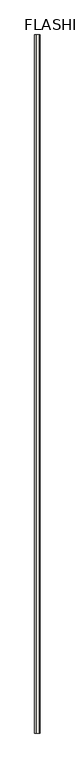
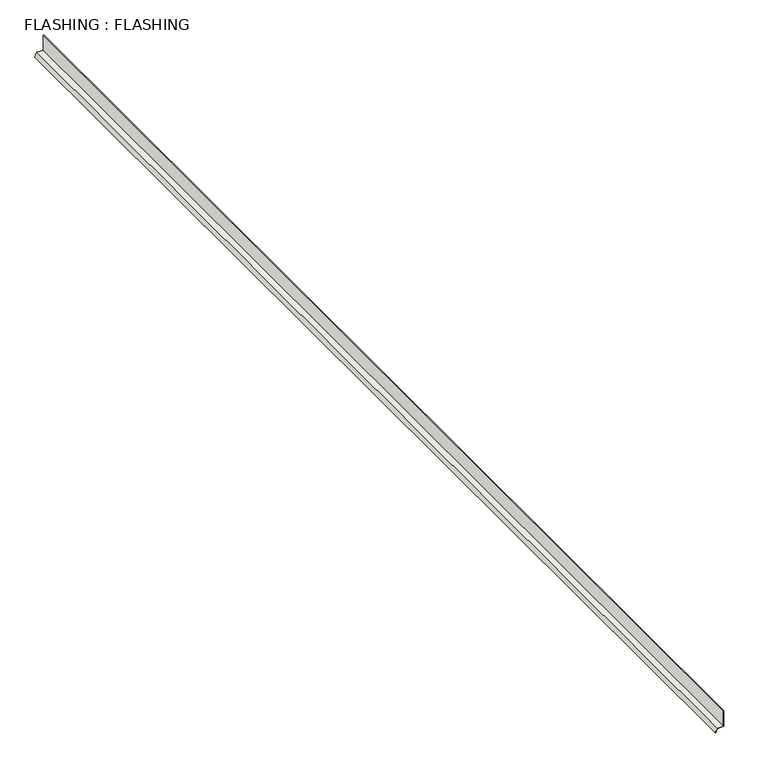
"""IFC4 building model written with IfcOpenShell, lengths in millimetres: wall geometry, FLASHING : FLASHING."""

from ifc_helpers import new_model, si_unit, frame, origin, place, context, project, spatial, polyline, outline, extrude, source, transform, mapped, element, save


def flashing_flashing_0e4c62f4(model_context):
    return source(origin(), model_context, "Body", "SweptSolid", [
        extrude(outline(polyline([(2162.175, 17920.4870052), (2210.3935166, 17920.4870052), (2210.3935166, 17918.8995052), (2163.7625, 17918.8995052), (2163.7625, 17900.4256562), (2151.3357976, 17894.6309897), (2150.6648911, 17896.0697533), (2162.175, 17901.4370052), (2162.175, 17920.4870052)])), frame((0.0, -3415.0384634, 0.0), z_axis=(0.0, 1.0, 0.0), x_axis=(0.0, 0.0, 1.0)), (0.0, 0.0, 1.0), 3403.6),
    ])


if __name__ == "__main__":
    model = new_model("IFC4")
    model_context = context("Model", 3, world=origin())
    ifc_project = project(units=[si_unit("LENGTHUNIT", "METRE", prefix="MILLI")], contexts=[model_context])
    site = spatial("IfcSite", under=ifc_project)
    building = spatial("IfcBuilding", under=site)
    placement = place(None, origin())
    flashing_flashing_shape = flashing_flashing_0e4c62f4(model_context)
    element("IfcWall", 1, ObjectType="FLASHING : FLASHING", at=placement, inside=building, context=model_context, shape_type="MappedRepresentation", body=[
        mapped(flashing_flashing_shape, transform((0.0, 0.0, 0.0), x_axis=(1.0, 0.0, 0.0), y_axis=(0.0, 1.0, 0.0), z_axis=(0.0, 0.0, 1.0))),
    ])
    save(model, "model.ifc")

# Revit data of these elements
# Element 1 (IfcWall, "FLASHING : FLASHING")
#   Materials on its faces: "FLASHING"
# Materials
#   "FLASHING": class "Metal", colour RGB 199 199 199, transparency 0, Description = "Carbon steel", Cost = 0
